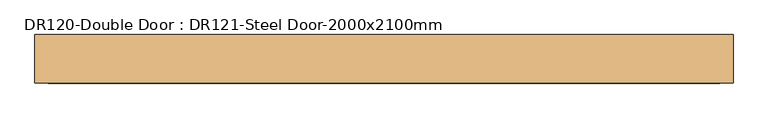
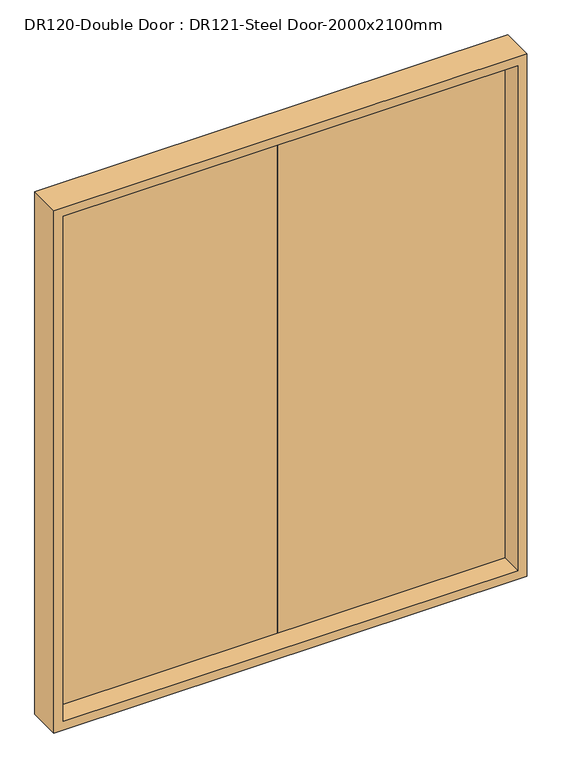
"""IFC4 building model written with IfcOpenShell, lengths in millimetres: door geometry, DR120-Double Door : DR121-Steel Door-2000x2100mm."""

from ifc_helpers import new_model, si_unit, frame, origin, place, context, project, spatial, polyline, outline, extrude, faceted_brep, source, transform, mapped, element, save


def dr120_double_door_dr121_steel_door_2000x2100mm_61964ec1(model_context):
    return source(origin(), model_context, "Body", "SolidModel", [
        extrude(outline(polyline([(880.0, 22.5), (0.0, 22.5), (0.0, 62.5), (880.0, 62.5), (880.0, 22.5)])), frame((0.0, 0.0, 20.0), z_axis=(0.0, 0.0, 1.0), x_axis=(1.0, 0.0, 0.0)), (0.0, 0.0, 1.0), 2060.0),
        extrude(outline(polyline([(0.0, 22.5), (-880.0, 22.5), (-880.0, 62.5), (0.0, 62.5), (0.0, 22.5)])), frame((0.0, 0.0, 20.0), z_axis=(0.0, 0.0, 1.0), x_axis=(1.0, 0.0, 0.0)), (0.0, 0.0, 1.0), 2060.0),
        faceted_brep([(900.0, -62.5, 2100.0), (900.0, 62.5, 2100.0), (-900.0, 62.5, 2100.0), (-900.0, -62.5, 2100.0), (865.0, 22.5, 2065.0), (865.0, -62.5, 2065.0), (-865.0, -62.5, 2065.0), (-865.0, 22.5, 2065.0), (880.0, 62.5, 2080.0), (880.0, 22.5, 2080.0), (-880.0, 22.5, 2080.0), (-880.0, 62.5, 2080.0), (-900.0, 62.5, 0.0), (-900.0, -62.5, 0.0), (-865.0, -62.5, 35.0), (-865.0, 22.5, 35.0), (-880.0, 22.5, 20.0), (-880.0, 62.5, 20.0), (900.0, 62.5, 0.0), (880.0, 62.5, 20.0), (900.0, -62.5, 0.0), (865.0, -62.5, 35.0), (865.0, 22.5, 35.0), (880.0, 22.5, 20.0)], [[[0, 1, 2, 3]], [[4, 5, 6, 7]], [[8, 9, 10, 11]], [[3, 2, 12, 13]], [[7, 6, 14, 15]], [[11, 10, 16, 17]], [[18, 12, 2, 1], [8, 11, 17, 19]], [[13, 12, 18, 20]], [[0, 3, 13, 20], [21, 14, 6, 5]], [[15, 14, 21, 22]], [[23, 16, 10, 9], [4, 7, 15, 22]], [[17, 16, 23, 19]], [[20, 18, 1, 0]], [[22, 21, 5, 4]], [[19, 23, 9, 8]]]),
    ])


if __name__ == "__main__":
    model = new_model("IFC4")
    model_context = context("Model", 3, world=origin())
    ifc_project = project(units=[si_unit("LENGTHUNIT", "METRE", prefix="MILLI")], contexts=[model_context])
    site = spatial("IfcSite", under=ifc_project)
    building = spatial("IfcBuilding", under=site)
    placement = place(None, origin())
    dr120_double_door_dr121_steel_door_2000x2100mm_shape = dr120_double_door_dr121_steel_door_2000x2100mm_61964ec1(model_context)
    element("IfcDoor", 1, ObjectType="DR120-Double Door : DR121-Steel Door-2000x2100mm", at=placement, inside=building, context=model_context, shape_type="MappedRepresentation", body=[
        mapped(dr120_double_door_dr121_steel_door_2000x2100mm_shape, transform((0.0, 0.0, 0.0), x_axis=(1.0, 0.0, 0.0), y_axis=(0.0, 1.0, 0.0), z_axis=(0.0, 0.0, 1.0))),
    ])
    save(model, "model.ifc")

# Revit data of these elements
# Type "DR120-Double Door : DR121-Steel Door-2000x2100mm"
#   Type Mark = "SD"
#   프레임 = ""
#   철물 = ""
#   유리/마감 = ""
#   위치/개소 = ""
#   부호 = "1/SD"
#   문번호 = ""
#   문기호 = "SD"
#   Analytic Construction = "<None>"
#   Height = 2100 mm
#   Width = 1800 mm
#   Define Thermal Properties by = 1
#   문 틀 = A04AQ098-00003_Steel Door_non FP_double
#   문 = 문
#   Function = (empty or 0)
#   Assembly Code = ""
#   Wall Closure = (empty or 0)
# Element 1 (IfcDoor, "DR120-Double Door : DR121-Steel Door-2000x2100mm")
#   Materials on its faces: "A04AQ098-00003_Steel Door_non FP_double", "문"
# Materials
#   "A04AQ098-00003_Steel Door_non FP_double": class "금속", colour RGB 247 247 247, transparency 0, Description = "Steel Door", W00) Work Master Code = "A04AQ098-00003", W01) Work Master_Lv1 = "Finishing Work", W02) Work Master_Lv2 = "Door & Window Work", W03) Work Master_Spec.1 = "Steel Door w/ Steel Frame", W04) Work Master_Spec.2 = "Fire Protective Rating: N/A, Double Door", W05) Work Master_Spec.3 = "w/ Hardware & Accessories", Cost = 0
#   "문": class "다양한", colour RGB 247 247 247, transparency 0
